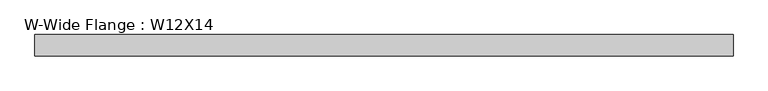
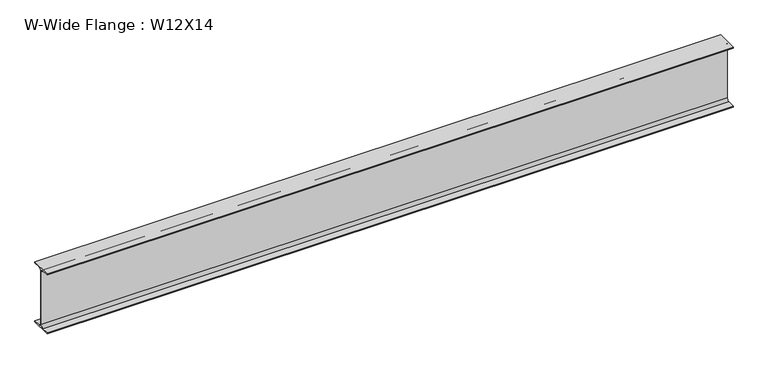
"""IFC4 building model written with IfcOpenShell, lengths in millimetres: beam geometry, W-Wide Flange : W12X14."""

from ifc_helpers import new_model, si_unit, point, frame, frame_2d, origin, place, context, project, spatial, polyline, circle_curve, trimmed, segment, composite_curve, outline, extrude, source, transform, mapped, element, save


def w_wide_flange_w12x14_d427c3bb(model_context):
    return source(origin(), model_context, "Body", "SweptSolid", [
        extrude(outline(composite_curve([segment(polyline([(50.419, -145.415), (50.419, -151.13), (-50.419, -151.13), (-50.419, -145.415), (-15.875, -145.415)]), True, "CONTINUOUS"), segment(trimmed(circle_curve(frame_2d((-15.875, -132.08)), 13.335), [point((-15.875, -145.415))], [point((-2.54, -132.08))], True, "CARTESIAN"), True, "CONTINUOUS"), segment(polyline([(-2.54, -132.08), (-2.54, 132.08)]), True, "CONTINUOUS"), segment(trimmed(circle_curve(frame_2d((-15.875, 132.08)), 13.335), [point((-2.54, 132.08))], [point((-15.875, 145.415))], True, "CARTESIAN"), True, "CONTINUOUS"), segment(polyline([(-15.875, 145.415), (-50.419, 145.415), (-50.419, 151.13), (50.419, 151.13), (50.419, 145.415), (15.875, 145.415)]), True, "CONTINUOUS"), segment(trimmed(circle_curve(frame_2d((15.875, 132.08)), 13.335), [point((15.875, 145.415))], [point((2.54, 132.08))], True, "CARTESIAN"), True, "CONTINUOUS"), segment(polyline([(2.54, 132.08), (2.54, -132.08)]), True, "CONTINUOUS"), segment(trimmed(circle_curve(frame_2d((15.875, -132.08)), 13.335), [point((2.54, -132.08))], [point((15.875, -145.415))], True, "CARTESIAN"), True, "CONTINUOUS"), segment(polyline([(15.875, -145.415), (50.419, -145.415)]), True, "CONTINUOUS")], self_intersect=False)), frame((-1586.072479, 0.0, 0.0), z_axis=(1.0, 0.0, 0.0), x_axis=(0.0, 1.0, 0.0)), (0.0, 0.0, 1.0), 3262.472479),
    ])


if __name__ == "__main__":
    model = new_model("IFC4")
    model_context = context("Model", 3, world=origin())
    ifc_project = project(units=[si_unit("LENGTHUNIT", "METRE", prefix="MILLI")], contexts=[model_context])
    site = spatial("IfcSite", under=ifc_project)
    building = spatial("IfcBuilding", under=site)
    placement = place(None, origin())
    w_wide_flange_w12x14_shape = w_wide_flange_w12x14_d427c3bb(model_context)
    element("IfcBeam", 1, ObjectType="W-Wide Flange : W12X14", at=placement, inside=building, context=model_context, shape_type="MappedRepresentation", body=[
        mapped(w_wide_flange_w12x14_shape, transform((0.0, 0.0, 0.0), x_axis=(1.0, 0.0, 0.0), y_axis=(0.0, 1.0, 0.0), z_axis=(0.0, 0.0, 1.0))),
    ])
    save(model, "model.ifc")

# Revit data of these elements
# Type "W-Wide Flange : W12X14"
#   Assembly Code = "B10"
#   W = 14
#   Length [instance default] = 5' - 0"
#   bf = 0' - 3.97"
#   d = 0' - 11.9"
#   k = 0' - 0 3/4"
#   k2 = 0' - 0.525"
#   tf = 0' - 0.225"
#   tw = 0' - 0.2"
#   A = 0.0288889 SF
#   Structural Material [instance default] = Steel ASTM A992
# Element 1 (IfcBeam, "W-Wide Flange : W12X14")
#   Materials on its faces: "Steel ASTM A992"
# Materials
#   "Steel ASTM A992": class "Metal", colour RGB 199 199 199, transparency 0, Description = "Structural steel 50ksi", Cost = 0
